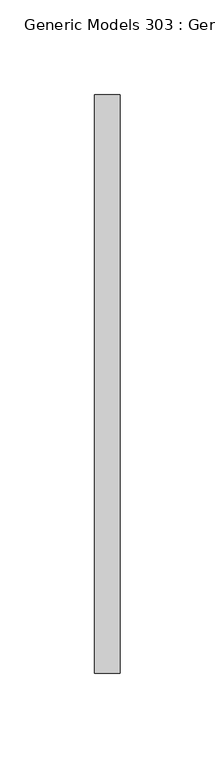
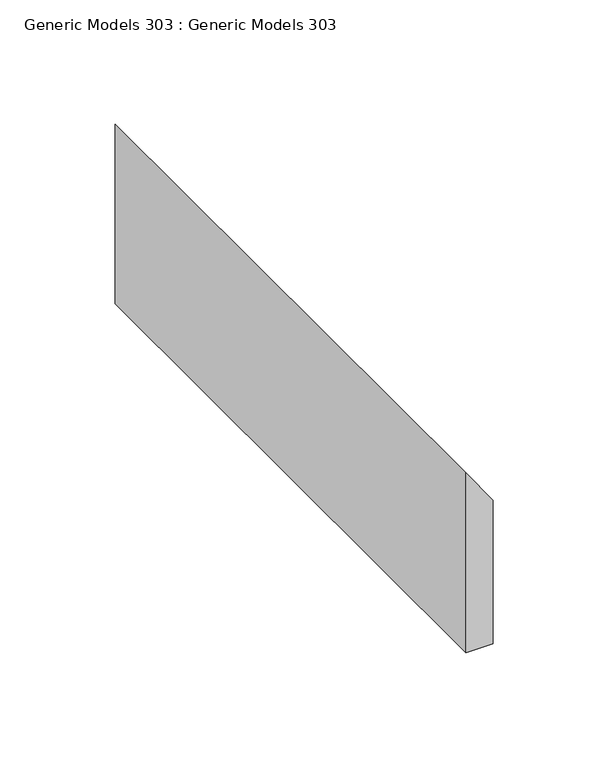
"""IFC4 building model written with IfcOpenShell, lengths in millimetres: proxy geometry, Generic Models 303 : Generic Models 303."""

from ifc_helpers import new_model, si_unit, frame, origin, place, context, project, spatial, polyline, outline, extrude, source, transform, mapped, element, save


def generic_models_303_generic_models_303_caacf8d9(model_context):
    return source(origin(), model_context, "Body", "SweptSolid", [
        extrude(outline(polyline([(124815.5645086, 4767.9223052), (124815.5645086, 4781.3763704), (124891.7645086, 4781.3763704), (124910.8145086, 4767.9223052), (124815.5645086, 4767.9223052)])), frame((0.0, 399.7309662, 0.0), z_axis=(0.0, 1.0, 0.0), x_axis=(0.0, 0.0, 1.0)), (0.0, 0.0, 1.0), 304.8),
    ])


if __name__ == "__main__":
    model = new_model("IFC4")
    model_context = context("Model", 3, world=origin())
    ifc_project = project(units=[si_unit("LENGTHUNIT", "METRE", prefix="MILLI")], contexts=[model_context])
    site = spatial("IfcSite", under=ifc_project)
    building = spatial("IfcBuilding", under=site)
    placement = place(None, origin())
    generic_models_303_generic_models_303_shape = generic_models_303_generic_models_303_caacf8d9(model_context)
    element("IfcBuildingElementProxy", 1, Name="Generic Models 303 : Generic Models 303", ObjectType="Generic Models 303 : Generic Models 303", at=placement, inside=building, context=model_context, shape_type="MappedRepresentation", body=[
        mapped(generic_models_303_generic_models_303_shape, transform((0.0, 0.0, 0.0), x_axis=(1.0, 0.0, 0.0), y_axis=(0.0, 1.0, 0.0), z_axis=(0.0, 0.0, 1.0))),
    ])
    save(model, "model.ifc")

# Revit data of these elements
# Element 1 (IfcBuildingElementProxy, "Generic Models 303 : Generic Models 303")
#   Materials on its faces: "_WOOD FLOORING (SPEC T.B.D.)"
# Materials
#   "_WOOD FLOORING (SPEC T.B.D.)": class "Generic", colour RGB 177 130 114, transparency 0, Cost = 0
